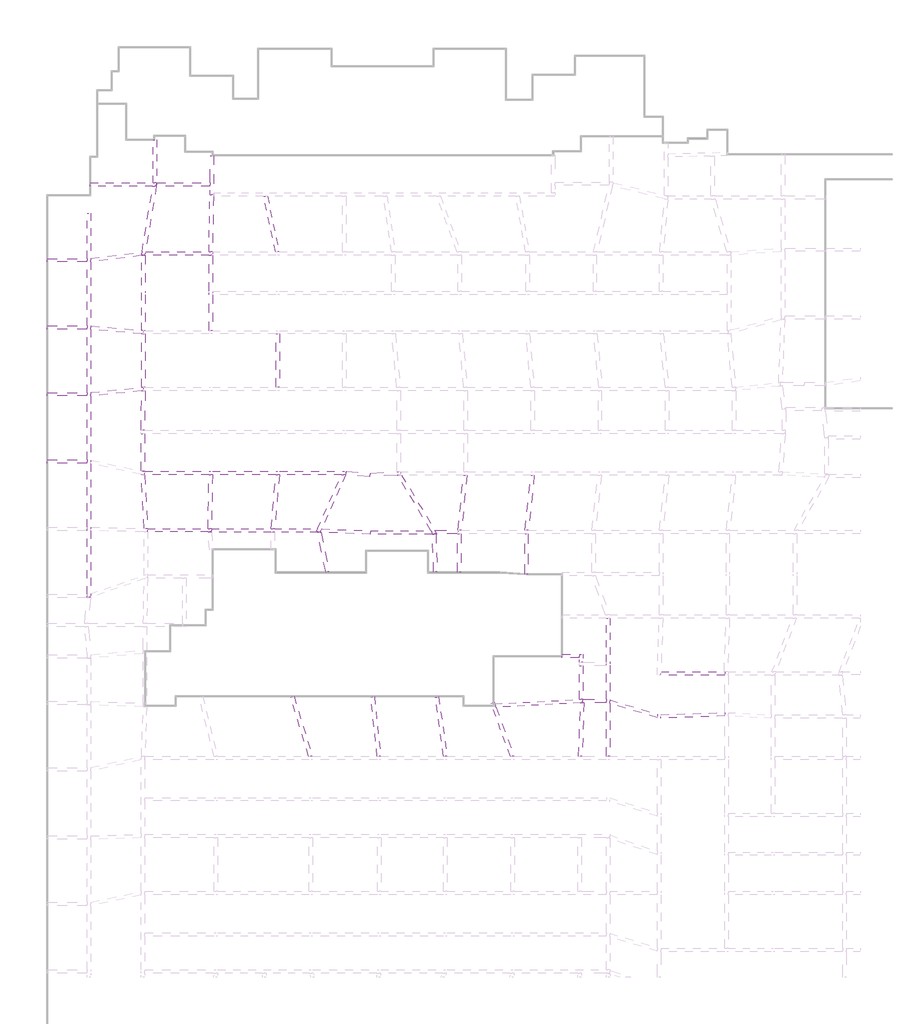
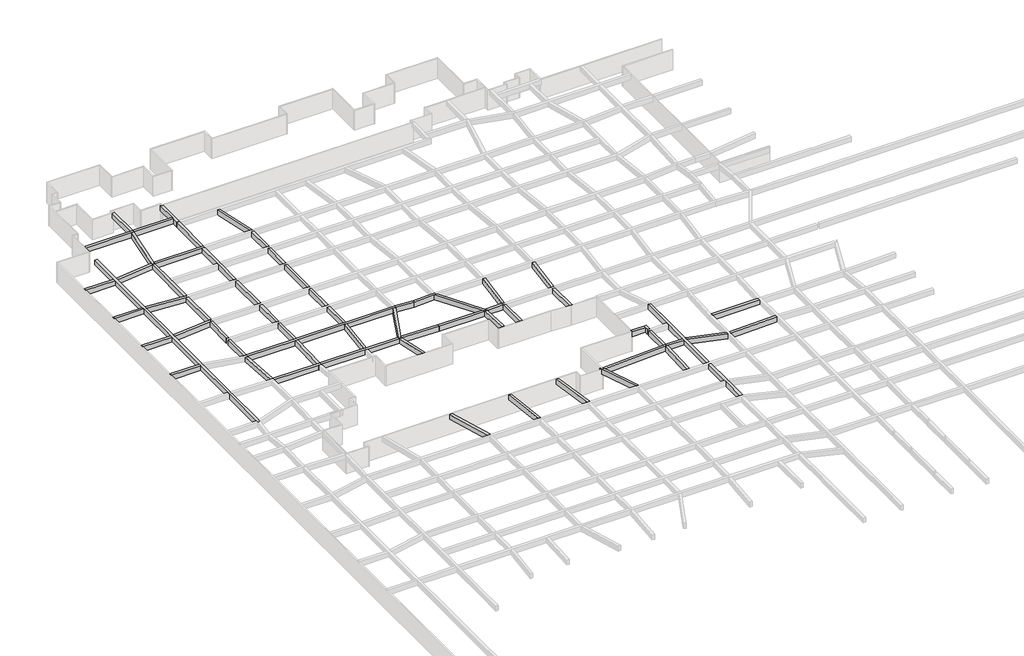
# One storey, part 35 of 45: 55 beams.
"""IFC4 building model written with IfcOpenShell, lengths in millimetres."""

from ifc_helpers import new_model, si_unit, frame, origin, place, context, project, spatial, polyline, outline, extrude, faceted_brep, element, save

model = new_model("IFC4")

# Units and contexts
model_context = context("Model", 3, world=origin())
ifc_project = project(units=[si_unit("LENGTHUNIT", "METRE", prefix="MILLI")], contexts=[model_context])

# Site, building, storey
site = spatial("IfcSite", under=ifc_project)
building = spatial("IfcBuilding", under=site)
storey = spatial("IfcBuildingStorey", under=building, Name="户型图", Elevation=0.0)

# Beams
placement = place(None, origin())
element("IfcBeam", 1, ObjectType="混凝土 - 矩形梁 : KL_beam", at=placement, inside=storey, context=model_context, shape_type="Brep", body=[
    faceted_brep([(-150040.5216564, 192731.9876735, 3300.0), (-150040.5216564, 192731.9876735, 2500.0), (-150040.5216564, 192331.9876735, 2500.0), (-150040.5216564, 192331.9876735, 3300.0), (-142370.8493457, 192331.9876735, 3300.0), (-142370.8493457, 192731.9876735, 3300.0), (-142740.5216564, 192731.9876735, 3300.0), (-142776.2701991, 192331.9876735, 3300.0), (-142370.8493457, 192331.9876735, 2500.0), (-142776.2701991, 192331.9876735, 2500.0), (-142370.8493457, 192731.9876735, 2500.0), (-142740.5216564, 192731.9876735, 2500.0)], [[[0, 1, 2, 3]], [[4, 5, 6, 0, 3, 7]], [[8, 4, 7, 3, 2, 9]], [[10, 8, 9, 2, 1, 11]], [[5, 10, 11, 1, 0, 6]], [[5, 4, 8, 10]]]),
])
element("IfcBeam", 2, ObjectType="混凝土 - 矩形梁 : KL_beam", at=placement, inside=storey, context=model_context, shape_type="Brep", body=[
    faceted_brep([(-143691.0021546, 184340.2921988, 3300.0), (-143624.9259227, 184740.2921988, 3300.0), (-142370.8493457, 192331.9876735, 3300.0), (-142776.2701991, 192331.9876735, 3300.0), (-144033.6062149, 184720.560815, 3300.0), (-144085.653783, 184405.4849301, 3300.0), (-143758.1300846, 184351.3811005, 3300.0), (-144085.653783, 184405.4849301, 2500.0), (-142776.2701991, 192331.9876735, 2500.0), (-144033.6062149, 184720.560815, 2500.0), (-142370.8493457, 192331.9876735, 2500.0), (-143624.9259227, 184740.2921988, 2500.0), (-143691.0021546, 184340.2921988, 2500.0), (-143758.1300846, 184351.3811005, 2500.0)], [[[0, 1, 2, 3, 4, 5, 6]], [[7, 5, 4, 3, 8, 9]], [[10, 11, 12, 13, 7, 9, 8]], [[2, 1, 0, 12, 11, 10]], [[3, 2, 10, 8]], [[0, 6, 5, 7, 13, 12]]]),
])
element("IfcBeam", 3, ObjectType="混凝土 - 矩形梁 : KL_beam", at=placement, inside=storey, context=model_context, shape_type="Brep", body=[
    faceted_brep([(-135864.1350128, 184340.2921988, 3300.0), (-135857.1529868, 184740.2921988, 3300.0), (-136257.213918, 184740.2921988, 3300.0), (-143624.9259227, 184740.2921988, 3300.0), (-143691.0021546, 184340.2921988, 3300.0), (-143669.0135418, 184340.2921988, 3300.0), (-136260.6744654, 184340.2921988, 3300.0), (-135864.1350128, 184340.2921988, 2500.0), (-143691.0021546, 184340.2921988, 2500.0), (-143669.0135418, 184340.2921988, 2500.0), (-136260.6744654, 184340.2921988, 2500.0), (-135857.1529868, 184740.2921988, 2500.0), (-143624.9259227, 184740.2921988, 2500.0), (-136257.213918, 184740.2921988, 2500.0)], [[[0, 1, 2, 3, 4, 5, 6]], [[7, 0, 6, 5, 4, 8, 9, 10]], [[11, 7, 10, 9, 8, 12, 13]], [[1, 11, 13, 12, 3, 2]], [[4, 3, 12, 8]], [[1, 0, 7, 11]]]),
])
element("IfcBeam", 4, ObjectType="混凝土 - 矩形梁 : KL_beam", at=placement, inside=storey, context=model_context, shape_type="Brep", body=[
    faceted_brep([(-135741.3000054, 191377.5050601, 3300.0), (-136141.3000054, 191380.9958072, 3300.0), (-136257.213918, 184740.2921988, 3300.0), (-135857.1529868, 184740.2921988, 3300.0), (-135744.7605527, 191179.2504337, 3300.0), (-135741.3000054, 191377.5050601, 2500.0), (-135857.1529868, 184740.2921988, 2500.0), (-135744.7605527, 191179.2504337, 2500.0), (-136141.3000054, 191380.9958072, 2500.0), (-136257.213918, 184740.2921988, 2500.0)], [[[0, 1, 2, 3, 4]], [[5, 0, 4, 3, 6, 7]], [[8, 5, 7, 6, 9]], [[1, 8, 9, 2]], [[3, 2, 9, 6]], [[1, 0, 5, 8]]]),
])
element("IfcBeam", 5, ObjectType="混凝土 - 矩形梁 : KL_beam", at=placement, inside=storey, context=model_context, shape_type="SweptSolid", body=[
    extrude(outline(polyline([(-128118.5648498, 184740.2921988), (-128527.5010878, 184740.2921988), (-129896.1439109, 191179.2504337), (-129487.2076729, 191179.2504337), (-128118.5648498, 184740.2921988)])), frame((0.0, 0.0, 2500.0), z_axis=(0.0, 0.0, 1.0), x_axis=(1.0, 0.0, 0.0)), (0.0, 0.0, 1.0), 800.0),
])
element("IfcBeam", 6, ObjectType="混凝土 - 矩形梁 : KL_beam", at=placement, inside=storey, context=model_context, shape_type="Brep", body=[
    faceted_brep([(-144085.653783, 184405.4849301, 3300.0), (-144033.6062149, 184720.560815, 3300.0), (-149980.0650049, 183990.4274835, 3300.0), (-149980.0650049, 183587.4235533, 3300.0), (-144069.0135418, 184313.2094117, 3300.0), (-143758.1300846, 184351.3811005, 3300.0), (-144033.6062149, 184720.560815, 2500.0), (-149980.0650049, 183990.4274835, 2500.0), (-144085.653783, 184405.4849301, 2500.0), (-143758.1300846, 184351.3811005, 2500.0), (-144069.0135418, 184313.2094117, 2500.0), (-149980.0650049, 183587.4235533, 2500.0)], [[[0, 1, 2, 3, 4, 5]], [[1, 6, 7, 2]], [[6, 8, 9, 10, 11, 7]], [[9, 5, 4, 3, 11, 10]], [[0, 8, 6, 1]], [[8, 0, 5, 9]], [[3, 2, 7, 11]]]),
])
element("IfcBeam", 7, ObjectType="混凝土 - 矩形梁 : KL_beam", at=placement, inside=storey, context=model_context, shape_type="Brep", body=[
    faceted_brep([(-149980.0650049, 189229.932653, 3300.0), (-149980.0650049, 189229.932653, 2500.0), (-150380.0650049, 189229.932653, 2500.0), (-150380.0650049, 189229.932653, 3300.0), (-150380.0650049, 144687.2740394, 3300.0), (-149980.0650049, 144687.2740394, 3300.0), (-149980.0650049, 145110.3223119, 3300.0), (-149980.0650049, 152424.9959274, 3300.0), (-149980.0650049, 152825.1148483, 3300.0), (-149980.0650049, 160182.9046895, 3300.0), (-149980.0650049, 160591.8409275, 3300.0), (-149980.0650049, 168048.193678, 3300.0), (-149980.0650049, 168450.028535, 3300.0), (-149980.0650049, 175746.0869301, 3300.0), (-149980.0650049, 176147.6148651, 3300.0), (-149980.0650049, 183587.4235533, 3300.0), (-149980.0650049, 183990.4274835, 3300.0), (-150380.0650049, 183964.3686062, 3300.0), (-150380.0650049, 183564.3686062, 3300.0), (-150380.0650049, 176164.3686062, 3300.0), (-150380.0650049, 175764.3686062, 3300.0), (-150380.0650049, 168429.932653, 3300.0), (-150380.0650049, 168029.932653, 3300.0), (-150380.0650049, 160629.932653, 3300.0), (-150380.0650049, 160229.932653, 3300.0), (-150380.0650049, 152829.932653, 3300.0), (-150380.0650049, 152429.932653, 3300.0), (-150380.0650049, 145029.932653, 3300.0), (-150380.0650049, 144687.2740394, 2500.0), (-150380.0650049, 183964.3686062, 2500.0), (-150380.0650049, 183564.3686062, 2500.0), (-150380.0650049, 176164.3686062, 2500.0), (-150380.0650049, 175764.3686062, 2500.0), (-150380.0650049, 168429.932653, 2500.0), (-150380.0650049, 168029.932653, 2500.0), (-150380.0650049, 160629.932653, 2500.0), (-150380.0650049, 160229.932653, 2500.0), (-150380.0650049, 152829.932653, 2500.0), (-150380.0650049, 152429.932653, 2500.0), (-150380.0650049, 145029.932653, 2500.0), (-149980.0650049, 144687.2740394, 2500.0), (-149980.0650049, 183990.4274835, 2500.0), (-149980.0650049, 183587.4235533, 2500.0), (-149980.0650049, 176147.6148651, 2500.0), (-149980.0650049, 175746.0869301, 2500.0), (-149980.0650049, 168450.028535, 2500.0), (-149980.0650049, 168048.193678, 2500.0), (-149980.0650049, 160591.8409275, 2500.0), (-149980.0650049, 160182.9046895, 2500.0), (-149980.0650049, 152825.1148483, 2500.0), (-149980.0650049, 152424.9959274, 2500.0), (-149980.0650049, 145110.3223119, 2500.0)], [[[0, 1, 2, 3]], [[4, 5, 6, 7, 8, 9, 10, 11, 12, 13, 14, 15, 16, 0, 3, 17, 18, 19, 20, 21, 22, 23, 24, 25, 26, 27]], [[28, 4, 27, 26, 25, 24, 23, 22, 21, 20, 19, 18, 17, 3, 2, 29, 30, 31, 32, 33, 34, 35, 36, 37, 38, 39]], [[40, 28, 39, 38, 37, 36, 35, 34, 33, 32, 31, 30, 29, 2, 1, 41, 42, 43, 44, 45, 46, 47, 48, 49, 50, 51]], [[5, 40, 51, 50, 49, 48, 47, 46, 45, 44, 43, 42, 41, 1, 0, 16, 15, 14, 13, 12, 11, 10, 9, 8, 7, 6]], [[5, 4, 28, 40]]]),
])
element("IfcBeam", 8, ObjectType="混凝土 - 矩形梁 : KL_beam", at=placement, inside=storey, context=model_context, shape_type="SweptSolid", body=[
    extrude(outline(polyline([(-155040.2933307, 183564.3686062), (-155040.2933307, 183964.3686062), (-150380.0650049, 183964.3686062), (-150380.0650049, 183564.3686062), (-155040.2933307, 183564.3686062)])), frame((0.0, 0.0, 2500.0), z_axis=(0.0, 0.0, 1.0), x_axis=(1.0, 0.0, 0.0)), (0.0, 0.0, 1.0), 800.0),
])
element("IfcBeam", 9, ObjectType="混凝土 - 矩形梁 : KL_beam", at=placement, inside=storey, context=model_context, shape_type="SweptSolid", body=[
    extrude(outline(polyline([(-155040.2933307, 175764.3686062), (-155040.2933307, 176164.3686062), (-150380.0650049, 176164.3686062), (-150380.0650049, 175764.3686062), (-155040.2933307, 175764.3686062)])), frame((0.0, 0.0, 2500.0), z_axis=(0.0, 0.0, 1.0), x_axis=(1.0, 0.0, 0.0)), (0.0, 0.0, 1.0), 800.0),
])
element("IfcBeam", 10, ObjectType="混凝土 - 矩形梁 : KL_beam", at=placement, inside=storey, context=model_context, shape_type="SweptSolid", body=[
    extrude(outline(polyline([(-155040.2933307, 168029.932653), (-155040.2933307, 168429.932653), (-150380.0650049, 168429.932653), (-150380.0650049, 168029.932653), (-155040.2933307, 168029.932653)])), frame((0.0, 0.0, 2500.0), z_axis=(0.0, 0.0, 1.0), x_axis=(1.0, 0.0, 0.0)), (0.0, 0.0, 1.0), 800.0),
])
element("IfcBeam", 11, ObjectType="混凝土 - 矩形梁 : KL_beam", at=placement, inside=storey, context=model_context, shape_type="SweptSolid", body=[
    extrude(outline(polyline([(-155040.2933307, 160229.932653), (-155040.2933307, 160629.932653), (-150380.0650049, 160629.932653), (-150380.0650049, 160229.932653), (-155040.2933307, 160229.932653)])), frame((0.0, 0.0, 2500.0), z_axis=(0.0, 0.0, 1.0), x_axis=(1.0, 0.0, 0.0)), (0.0, 0.0, 1.0), 800.0),
])
element("IfcBeam", 12, ObjectType="混凝土 - 矩形梁 : KL_beam", at=placement, inside=storey, context=model_context, shape_type="Brep", body=[
    faceted_brep([(-143913.3828558, 175215.3210168, 3300.0), (-143895.9184786, 175615.3210168, 3300.0), (-144069.0135418, 175630.4648726, 3300.0), (-149980.0650049, 176147.6148651, 3300.0), (-149980.0650049, 175746.0869301, 3300.0), (-144069.0135418, 175228.9369376, 3300.0), (-143913.3828558, 175215.3210168, 2500.0), (-149980.0650049, 175746.0869301, 2500.0), (-144069.0135418, 175228.9369376, 2500.0), (-143895.9184786, 175615.3210168, 2500.0), (-149980.0650049, 176147.6148651, 2500.0), (-144069.0135418, 175630.4648726, 2500.0)], [[[0, 1, 2, 3, 4, 5]], [[6, 0, 5, 4, 7, 8]], [[9, 6, 8, 7, 10, 11]], [[1, 9, 11, 10, 3, 2]], [[4, 3, 10, 7]], [[1, 0, 6, 9]]]),
])
element("IfcBeam", 13, ObjectType="混凝土 - 矩形梁 : KL_beam", at=placement, inside=storey, context=model_context, shape_type="Brep", body=[
    faceted_brep([(-143859.4474089, 168635.1135794, 3300.0), (-143878.581976, 169035.1135794, 3300.0), (-144069.0135418, 169016.8526647, 3300.0), (-149980.0650049, 168450.028535, 3300.0), (-149980.0650049, 168048.193678, 3300.0), (-144071.7625624, 168614.7541979, 3300.0), (-143859.4474089, 168635.1135794, 2500.0), (-149980.0650049, 168048.193678, 2500.0), (-144071.7625624, 168614.7541979, 2500.0), (-143878.581976, 169035.1135794, 2500.0), (-149980.0650049, 168450.028535, 2500.0), (-144069.0135418, 169016.8526647, 2500.0)], [[[0, 1, 2, 3, 4, 5]], [[6, 0, 5, 4, 7, 8]], [[9, 6, 8, 7, 10, 11]], [[1, 9, 11, 10, 3, 2]], [[4, 3, 10, 7]], [[1, 0, 6, 9]]]),
])
element("IfcBeam", 14, ObjectType="混凝土 - 矩形梁 : KL_beam", at=placement, inside=storey, context=model_context, shape_type="Brep", body=[
    faceted_brep([(-143391.7428195, 152664.4498776, 3300.0), (-143391.9766848, 152669.0307398, 3300.0), (-143707.512981, 158849.6325984, 3300.0), (-144112.4278844, 158935.6999181, 3300.0), (-143792.7630206, 152674.2292868, 3300.0), (-144112.4278844, 158935.6999181, 2500.0), (-143792.7630206, 152674.2292868, 2500.0), (-143707.512981, 158849.6325984, 2500.0), (-143391.9766848, 152669.0307398, 2500.0), (-143391.7428195, 152664.4498776, 2500.0)], [[[0, 1, 2, 3, 4]], [[3, 5, 6, 4]], [[7, 8, 9, 6, 5]], [[2, 1, 0, 9, 8, 7]], [[3, 2, 7, 5]], [[0, 4, 6, 9]]]),
])
element("IfcBeam", 15, ObjectType="混凝土 - 矩形梁 : KL_beam", at=placement, inside=storey, context=model_context, shape_type="Brep", body=[
    faceted_brep([(-143391.9766848, 152669.0307398, 3300.0), (-143391.7428195, 152664.4498776, 3300.0), (-143382.0266166, 152664.2129351, 3300.0), (-143382.0266166, 152269.0307398, 3300.0), (-136378.8977394, 152269.0307398, 3300.0), (-135978.8368082, 152269.0307398, 3300.0), (-135972.5274142, 152630.4956807, 3300.0), (-135971.8547822, 152669.0307398, 3300.0), (-136371.9157134, 152669.0307398, 3300.0), (-135978.8368082, 152269.0307398, 2500.0), (-143382.0266166, 152269.0307398, 2500.0), (-136378.8977394, 152269.0307398, 2500.0), (-143391.7428195, 152664.4498776, 2500.0), (-143391.9766848, 152669.0307398, 2500.0), (-136371.9157134, 152669.0307398, 2500.0), (-135971.8547822, 152669.0307398, 2500.0), (-135972.5274142, 152630.4956807, 2500.0), (-143382.0266166, 152664.2129351, 2500.0)], [[[0, 1, 2, 3, 4, 5, 6, 7, 8]], [[9, 5, 4, 3, 10, 11]], [[12, 13, 14, 15, 16, 9, 11, 10, 17]], [[13, 0, 8, 7, 15, 14]], [[1, 0, 13, 12]], [[2, 17, 10, 3]], [[17, 2, 1, 12]], [[7, 6, 5, 9, 16, 15]]]),
])
element("IfcBeam", 16, ObjectType="混凝土 - 矩形梁 : KL_beam", at=placement, inside=storey, context=model_context, shape_type="Brep", body=[
    faceted_brep([(-135860.6744654, 184340.2921988, 3300.0), (-135864.1350128, 184340.2921988, 3300.0), (-136260.6744654, 184340.2921988, 3300.0), (-136260.6744654, 180177.2946529, 3300.0), (-136260.6744654, 179777.2946529, 3300.0), (-136260.6744654, 175615.3210168, 3300.0), (-135860.6744654, 175615.3210168, 3300.0), (-135860.6744654, 179777.2946529, 3300.0), (-135860.6744654, 180177.2946529, 3300.0), (-136260.6744654, 184340.2921988, 2500.0), (-136260.6744654, 180177.2946529, 2500.0), (-136260.6744654, 179777.2946529, 2500.0), (-136260.6744654, 175615.3210168, 2500.0), (-135864.1350128, 184340.2921988, 2500.0), (-135860.6744654, 184340.2921988, 2500.0), (-135860.6744654, 180177.2946529, 2500.0), (-135860.6744654, 179777.2946529, 2500.0), (-135860.6744654, 175615.3210168, 2500.0)], [[[0, 1, 2, 3, 4, 5, 6, 7, 8]], [[2, 9, 10, 11, 12, 5, 4, 3]], [[9, 13, 14, 15, 16, 17, 12, 11, 10]], [[14, 0, 8, 7, 6, 17, 16, 15]], [[9, 2, 1, 0, 14, 13]], [[6, 5, 12, 17]]]),
    faceted_brep([(-136260.6744654, 175215.3210168, 3300.0), (-135860.6744654, 175215.3210168, 3300.0), (-135860.6744654, 175215.3210168, 2500.0), (-136260.6744654, 175215.3210168, 2500.0), (-135860.6744654, 169035.1135794, 3300.0), (-136260.6744654, 169035.1135794, 3300.0), (-136260.6744654, 169035.1135794, 2500.0), (-135860.6744654, 169035.1135794, 2500.0)], [[[0, 1, 2, 3]], [[4, 5, 6, 7]], [[1, 0, 5, 4]], [[0, 3, 6, 5]], [[3, 2, 7, 6]], [[2, 1, 4, 7]]]),
    faceted_brep([(-135860.6744654, 168635.1135794, 3300.0), (-136260.6744654, 168635.1135794, 3300.0), (-136260.6744654, 164050.6823883, 3300.0), (-135860.6744654, 164050.6823883, 3300.0), (-136260.6744654, 168635.1135794, 2500.0), (-136260.6744654, 164050.6823883, 2500.0), (-135860.6744654, 168635.1135794, 2500.0), (-135860.6744654, 164050.6823883, 2500.0)], [[[0, 1, 2, 3]], [[1, 4, 5, 2]], [[4, 6, 7, 5]], [[6, 0, 3, 7]], [[1, 0, 6, 4]], [[3, 2, 5, 7]]]),
    faceted_brep([(-136260.6744654, 163650.6823883, 3300.0), (-135860.6744654, 163650.6823883, 3300.0), (-135860.6744654, 163650.6823883, 2500.0), (-136260.6744654, 163650.6823883, 2500.0), (-136260.6744654, 159299.3775215, 3300.0), (-135860.6744654, 159299.3775215, 3300.0), (-136260.6744654, 159299.3775215, 2500.0), (-135860.6744654, 159299.3775215, 2500.0)], [[[0, 1, 2, 3]], [[1, 0, 4, 5]], [[0, 3, 6, 4]], [[3, 2, 7, 6]], [[2, 1, 5, 7]], [[5, 4, 6, 7]]]),
])
element("IfcBeam", 17, ObjectType="混凝土 - 矩形梁 : KL_beam", at=placement, inside=storey, context=model_context, shape_type="SweptSolid", body=[
    extrude(outline(polyline([(-135971.8547822, 152669.0307398), (-136371.9157134, 152669.0307398), (-136263.1646058, 158899.3775215), (-135863.1036746, 158899.3775215), (-135971.8547822, 152669.0307398)])), frame((0.0, 0.0, 2500.0), z_axis=(0.0, 0.0, 1.0), x_axis=(1.0, 0.0, 0.0)), (0.0, 0.0, 1.0), 800.0),
])
element("IfcBeam", 18, ObjectType="混凝土 - 矩形梁 : KL_beam", at=placement, inside=storey, context=model_context, shape_type="Brep", body=[
    faceted_brep([(-143899.5027499, 159299.3775215, 3300.0), (-143728.6193094, 159263.055125, 3300.0), (-143710.0525927, 158899.3775215, 3300.0), (-136263.1646058, 158899.3775215, 3300.0), (-135863.1036746, 158899.3775215, 3300.0), (-128498.7833567, 158899.3775215, 3300.0), (-128097.2554216, 158899.3775215, 3300.0), (-120868.6474581, 158899.3775215, 3300.0), (-120430.7929467, 158899.3775215, 3300.0), (-120360.6744654, 159056.8662092, 3300.0), (-120360.6744654, 159285.8508502, 3300.0), (-120360.6744654, 159299.3775215, 3300.0), (-120760.6744654, 159299.3775215, 3300.0), (-128080.5216564, 159299.3775215, 3300.0), (-128480.5216564, 159299.3775215, 3300.0), (-135860.6744654, 159299.3775215, 3300.0), (-136260.6744654, 159299.3775215, 3300.0), (-143730.8224936, 159299.3775215, 3300.0), (-143710.0525927, 158899.3775215, 2500.0), (-136263.1646058, 158899.3775215, 2500.0), (-135863.1036746, 158899.3775215, 2500.0), (-128498.7833567, 158899.3775215, 2500.0), (-128097.2554216, 158899.3775215, 2500.0), (-120868.6474581, 158899.3775215, 2500.0), (-120430.7929467, 158899.3775215, 2500.0), (-143728.6193094, 159263.055125, 2500.0), (-143899.5027499, 159299.3775215, 2500.0), (-143730.8224936, 159299.3775215, 2500.0), (-136260.6744654, 159299.3775215, 2500.0), (-135860.6744654, 159299.3775215, 2500.0), (-128480.5216564, 159299.3775215, 2500.0), (-128080.5216564, 159299.3775215, 2500.0), (-120760.6744654, 159299.3775215, 2500.0), (-120360.6744654, 159299.3775215, 2500.0), (-120360.6744654, 159285.8508502, 2500.0), (-120360.6744654, 159056.8662092, 2500.0)], [[[0, 1, 2, 3, 4, 5, 6, 7, 8, 9, 10, 11, 12, 13, 14, 15, 16, 17]], [[2, 18, 19, 20, 21, 22, 23, 24, 8, 7, 6, 5, 4, 3]], [[25, 26, 27, 28, 29, 30, 31, 32, 33, 34, 35, 24, 23, 22, 21, 20, 19, 18]], [[26, 0, 17, 16, 15, 14, 13, 12, 11, 33, 32, 31, 30, 29, 28, 27]], [[25, 1, 0, 26]], [[1, 25, 18, 2]], [[11, 10, 9, 35, 34, 33]], [[35, 9, 8, 24]]]),
])
element("IfcBeam", 19, ObjectType="混凝土 - 矩形梁 : KL_beam", at=placement, inside=storey, context=model_context, shape_type="SweptSolid", body=[
    extrude(outline(polyline([(-144130.8224936, 163650.6823883), (-143730.8224936, 163650.6823883), (-143730.8224936, 159299.3775215), (-143899.5027499, 159299.3775215), (-144130.8224936, 159348.5460509), (-144130.8224936, 163650.6823883)])), frame((0.0, 0.0, 2500.0), z_axis=(0.0, 0.0, 1.0), x_axis=(1.0, 0.0, 0.0)), (0.0, 0.0, 1.0), 800.0),
])
element("IfcBeam", 20, ObjectType="混凝土 - 矩形梁 : KL_beam", at=placement, inside=storey, context=model_context, shape_type="SweptSolid", body=[
    extrude(outline(polyline([(-144071.7625624, 168614.7541979), (-143859.4474089, 168635.1135794), (-143671.4793509, 168635.1135794), (-143728.3270835, 164050.6823883), (-144128.3578352, 164050.6823883), (-144071.7625624, 168614.7541979)])), frame((0.0, 0.0, 2500.0), z_axis=(0.0, 0.0, 1.0), x_axis=(1.0, 0.0, 0.0)), (0.0, 0.0, 1.0), 800.0),
])
element("IfcBeam", 21, ObjectType="混凝土 - 矩形梁 : KL_beam", at=placement, inside=storey, context=model_context, shape_type="Brep", body=[
    faceted_brep([(-143878.581976, 169035.1135794, 3300.0), (-143669.0135418, 169035.1135794, 3300.0), (-143669.0135418, 175215.3210168, 3300.0), (-143913.3828558, 175215.3210168, 3300.0), (-144069.0135418, 175228.9369376, 3300.0), (-144069.0135418, 169016.8526647, 3300.0), (-144066.7738093, 169017.0674377, 3300.0), (-143669.0135418, 169035.1135794, 2500.0), (-143669.0135418, 175215.3210168, 2500.0), (-143878.581976, 169035.1135794, 2500.0), (-144066.7738093, 169017.0674377, 2500.0), (-144069.0135418, 169016.8526647, 2500.0), (-144069.0135418, 175228.9369376, 2500.0), (-143913.3828558, 175215.3210168, 2500.0)], [[[0, 1, 2, 3, 4, 5, 6]], [[1, 7, 8, 2]], [[7, 9, 10, 11, 12, 13, 8]], [[4, 12, 11, 5]], [[1, 0, 9, 7]], [[3, 2, 8, 13]], [[4, 3, 13, 12]], [[5, 11, 10, 9, 0, 6]]]),
])
element("IfcBeam", 22, ObjectType="混凝土 - 矩形梁 : KL_beam", at=placement, inside=storey, context=model_context, shape_type="Brep", body=[
    faceted_brep([(-143895.9184786, 175615.3210168, 3300.0), (-143669.0135418, 175615.3210168, 3300.0), (-143669.0135418, 179777.2946529, 3300.0), (-143669.0135418, 180177.2946529, 3300.0), (-143669.0135418, 184340.2921988, 3300.0), (-143691.0021546, 184340.2921988, 3300.0), (-143758.1300846, 184351.3811005, 3300.0), (-144069.0135418, 184313.2094117, 3300.0), (-144069.0135418, 175630.4648726, 3300.0), (-143669.0135418, 175615.3210168, 2500.0), (-143669.0135418, 179777.2946529, 2500.0), (-143669.0135418, 180177.2946529, 2500.0), (-143669.0135418, 184340.2921988, 2500.0), (-143895.9184786, 175615.3210168, 2500.0), (-144069.0135418, 175630.4648726, 2500.0), (-144069.0135418, 184313.2094117, 2500.0), (-143758.1300846, 184351.3811005, 2500.0), (-143691.0021546, 184340.2921988, 2500.0)], [[[0, 1, 2, 3, 4, 5, 6, 7, 8]], [[1, 9, 10, 11, 12, 4, 3, 2]], [[9, 13, 14, 15, 16, 17, 12, 11, 10]], [[7, 15, 14, 8]], [[1, 0, 13, 9]], [[15, 7, 6, 16]], [[6, 5, 17, 16]], [[5, 4, 12, 17]], [[0, 8, 14, 13]]]),
])
element("IfcBeam", 23, ObjectType="混凝土 - 矩形梁 : KL_beam", at=placement, inside=storey, context=model_context, shape_type="SweptSolid", body=[
    extrude(outline(polyline([(-128480.5216564, 184340.2921988), (-128080.5216564, 184340.2921988), (-128080.5216564, 180177.2946529), (-128480.5216564, 180177.2946529), (-128480.5216564, 184340.2921988)])), frame((0.0, 0.0, 2500.0), z_axis=(0.0, 0.0, 1.0), x_axis=(1.0, 0.0, 0.0)), (0.0, 0.0, 1.0), 800.0),
    extrude(outline(polyline([(-128080.5216564, 159299.3775215), (-128480.5216564, 159299.3775215), (-128480.5216564, 163650.6823883), (-128080.5216564, 163650.6823883), (-128080.5216564, 159299.3775215)])), frame((0.0, 0.0, 2500.0), z_axis=(0.0, 0.0, 1.0), x_axis=(1.0, 0.0, 0.0)), (0.0, 0.0, 1.0), 800.0),
    extrude(outline(polyline([(-128480.5216564, 175215.3210168), (-128080.5216564, 175215.3210168), (-128080.5216564, 169035.1135794), (-128480.5216564, 169035.1135794), (-128480.5216564, 175215.3210168)])), frame((0.0, 0.0, 2500.0), z_axis=(0.0, 0.0, 1.0), x_axis=(1.0, 0.0, 0.0)), (0.0, 0.0, 1.0), 800.0),
    extrude(outline(polyline([(-128080.5216564, 175615.3210168), (-128480.5216564, 175615.3210168), (-128480.5216564, 179777.2946529), (-128080.5216564, 179777.2946529), (-128080.5216564, 175615.3210168)])), frame((0.0, 0.0, 2500.0), z_axis=(0.0, 0.0, 1.0), x_axis=(1.0, 0.0, 0.0)), (0.0, 0.0, 1.0), 800.0),
    extrude(outline(polyline([(-128480.5216564, 168635.1135794), (-128080.5216564, 168635.1135794), (-128080.5216564, 164050.6823883), (-128480.5216564, 164050.6823883), (-128480.5216564, 168635.1135794)])), frame((0.0, 0.0, 2500.0), z_axis=(0.0, 0.0, 1.0), x_axis=(1.0, 0.0, 0.0)), (0.0, 0.0, 1.0), 800.0),
])
element("IfcBeam", 24, ObjectType="混凝土 - 矩形梁 : KL_beam", at=placement, inside=storey, context=model_context, shape_type="SweptSolid", body=[
    extrude(outline(polyline([(-128498.7833567, 158899.3775215), (-128097.2554216, 158899.3775215), (-128645.7115157, 152630.4956807), (-129047.2394507, 152630.4956807), (-128498.7833567, 158899.3775215)])), frame((0.0, 0.0, 2500.0), z_axis=(0.0, 0.0, 1.0), x_axis=(1.0, 0.0, 0.0)), (0.0, 0.0, 1.0), 800.0),
])
element("IfcBeam", 25, ObjectType="混凝土 - 矩形梁 : KL_beam", at=placement, inside=storey, context=model_context, shape_type="Brep", body=[
    faceted_brep([(-123767.4305173, 152388.604171, 3300.0), (-123412.3130339, 152230.4956807, 3300.0), (-123402.0123343, 152225.9095138, 3300.0), (-123226.540494, 152620.0257198, 3300.0), (-120434.9382056, 158890.0671176, 3300.0), (-120430.7929467, 158899.3775215, 3300.0), (-120868.6474581, 158899.3775215, 3300.0), (-123659.7334785, 152630.4956807, 3300.0), (-123767.4305173, 152388.604171, 2500.0), (-120868.6474581, 158899.3775215, 2500.0), (-123659.7334785, 152630.4956807, 2500.0), (-123402.0123343, 152225.9095138, 2500.0), (-123412.3130339, 152230.4956807, 2500.0), (-120430.7929467, 158899.3775215, 2500.0), (-120434.9382056, 158890.0671176, 2500.0), (-123226.540494, 152620.0257198, 2500.0)], [[[0, 1, 2, 3, 4, 5, 6, 7]], [[8, 0, 7, 6, 9, 10]], [[11, 12, 8, 10, 9, 13, 14, 15]], [[2, 11, 15, 14, 13, 5, 4, 3]], [[6, 5, 13, 9]], [[2, 1, 0, 8, 12, 11]]]),
])
element("IfcBeam", 26, ObjectType="混凝土 - 矩形梁 : KL_beam", at=placement, inside=storey, context=model_context, shape_type="Brep", body=[
    faceted_brep([(-117566.6583118, 159090.4742081, 3300.0), (-120360.6744654, 159285.8508502, 3300.0), (-120360.6744654, 159056.8662092, 3300.0), (-120430.7929467, 158899.3775215, 3300.0), (-120434.9382056, 158890.0671176, 3300.0), (-117570.1554489, 158689.7419925, 3300.0), (-120434.9382056, 158890.0671176, 2500.0), (-117570.1554489, 158689.7419925, 2500.0), (-120430.7929467, 158899.3775215, 2500.0), (-120360.6744654, 159056.8662092, 2500.0), (-120360.6744654, 159285.8508502, 2500.0), (-117566.6583118, 159090.4742081, 2500.0)], [[[0, 1, 2, 3, 4, 5]], [[5, 4, 6, 7]], [[7, 6, 8, 9, 10, 11]], [[1, 0, 11, 10]], [[2, 9, 8, 6, 4, 3]], [[9, 2, 1, 10]], [[0, 5, 7, 11]]]),
])
element("IfcBeam", 27, ObjectType="混凝土 - 矩形梁 : KL_beam", at=placement, inside=storey, context=model_context, shape_type="Brep", body=[
    faceted_brep([(-117566.6583118, 159090.4742081, 3300.0), (-117570.1554489, 158689.7419925, 3300.0), (-114382.4696565, 158856.8015259, 3300.0), (-114259.4336062, 158863.2495721, 3300.0), (-114072.9294157, 158873.0238425, 3300.0), (-114072.9294157, 159263.2495721, 3300.0), (-114072.9294157, 159273.5727809, 3300.0), (-114472.9294157, 159252.6096692, 3300.0), (-117570.1554489, 158689.7419925, 2500.0), (-114382.4696565, 158856.8015259, 2500.0), (-114259.4336062, 158863.2495721, 2500.0), (-114072.9294157, 158873.0238425, 2500.0), (-117566.6583118, 159090.4742081, 2500.0), (-114472.9294157, 159252.6096692, 2500.0), (-114072.9294157, 159273.5727809, 2500.0), (-114072.9294157, 159263.2495721, 2500.0)], [[[0, 1, 2, 3, 4, 5, 6, 7]], [[1, 8, 9, 10, 11, 4, 3, 2]], [[8, 12, 13, 14, 15, 11, 10, 9]], [[12, 0, 7, 6, 14, 13]], [[0, 12, 8, 1]], [[6, 5, 4, 11, 15, 14]]]),
])
element("IfcBeam", 28, ObjectType="混凝土 - 矩形梁 : KL_beam", at=placement, inside=storey, context=model_context, shape_type="Brep", body=[
    faceted_brep([(-110310.4324421, 152079.7935386, 3300.0), (-109843.7790832, 152079.7935386, 3300.0), (-110084.1233308, 152479.7935386, 3300.0), (-113919.6906746, 158863.2495721, 3300.0), (-114259.4336062, 158863.2495721, 3300.0), (-114382.4696565, 158856.8015259, 3300.0), (-110515.509273, 152421.0987005, 3300.0), (-114382.4696565, 158856.8015259, 2500.0), (-110515.509273, 152421.0987005, 2500.0), (-110310.4324421, 152079.7935386, 2500.0), (-109843.7790832, 152079.7935386, 2500.0), (-114259.4336062, 158863.2495721, 2500.0), (-113919.6906746, 158863.2495721, 2500.0), (-110084.1233308, 152479.7935386, 2500.0)], [[[0, 1, 2, 3, 4, 5, 6]], [[5, 7, 8, 9, 0, 6]], [[10, 9, 8, 7, 11, 12, 13]], [[1, 10, 13, 12, 3, 2]], [[7, 5, 4, 11]], [[4, 3, 12, 11]], [[1, 0, 9, 10]]]),
])
element("IfcBeam", 29, ObjectType="混凝土 - 矩形梁 : KL_beam", at=placement, inside=storey, context=model_context, shape_type="Brep", body=[
    faceted_brep([(-110084.1233308, 152479.7935386, 3300.0), (-109843.7790832, 152079.7935386, 3300.0), (-107419.2456688, 152079.7935386, 3300.0), (-107399.1449794, 152079.7935386, 3300.0), (-107399.1449794, 152479.7935386, 3300.0), (-110084.1233308, 152479.7935386, 2500.0), (-107399.1449794, 152479.7935386, 2500.0), (-109843.7790832, 152079.7935386, 2500.0), (-107399.1449794, 152079.7935386, 2500.0), (-107419.2456688, 152079.7935386, 2500.0)], [[[0, 1, 2, 3, 4]], [[5, 0, 4, 6]], [[7, 5, 6, 8, 9]], [[1, 7, 9, 8, 3, 2]], [[1, 0, 5, 7]], [[4, 3, 8, 6]]]),
])
element("IfcBeam", 30, ObjectType="混凝土 - 矩形梁 : KL_beam", at=placement, inside=storey, context=model_context, shape_type="SweptSolid", body=[
    extrude(outline(polyline([(-106996.9062488, 152479.7935386), (-107399.1449794, 152479.7935386), (-106722.8306205, 158863.2495721), (-106320.5918899, 158863.2495721), (-106996.9062488, 152479.7935386)])), frame((0.0, 0.0, 2500.0), z_axis=(0.0, 0.0, 1.0), x_axis=(1.0, 0.0, 0.0)), (0.0, 0.0, 1.0), 800.0),
])
element("IfcBeam", 31, ObjectType="混凝土 - 矩形梁 : KL_beam", at=placement, inside=storey, context=model_context, shape_type="SweptSolid", body=[
    extrude(outline(polyline([(-98947.1541949, 158863.2495721), (-98544.9154643, 158863.2495721), (-99221.2298232, 152479.7935386), (-99623.4685538, 152479.7935386), (-98947.1541949, 158863.2495721)])), frame((0.0, 0.0, 2500.0), z_axis=(0.0, 0.0, 1.0), x_axis=(1.0, 0.0, 0.0)), (0.0, 0.0, 1.0), 800.0),
])
element("IfcBeam", 32, ObjectType="混凝土 - 矩形梁 : KL_beam", at=placement, inside=storey, context=model_context, shape_type="Brep", body=[
    faceted_brep([(-123402.0123343, 152225.9095138, 3300.0), (-123281.0986767, 152221.6871158, 3300.0), (-117536.9980107, 152021.0987005, 3300.0), (-117530.0159847, 152421.0987005, 3300.0), (-123226.540494, 152620.0257198, 3300.0), (-123402.0123343, 152225.9095138, 2500.0), (-123281.0986767, 152221.6871158, 2500.0), (-117536.9980107, 152021.0987005, 2500.0), (-123226.540494, 152620.0257198, 2500.0), (-117530.0159847, 152421.0987005, 2500.0)], [[[0, 1, 2, 3, 4]], [[2, 1, 0, 5, 6, 7]], [[7, 6, 5, 8, 9]], [[3, 9, 8, 4]], [[0, 4, 8, 5]], [[3, 2, 7, 9]]]),
])
element("IfcBeam", 33, ObjectType="混凝土 - 矩形梁 : KL_beam", at=placement, inside=storey, context=model_context, shape_type="Brep", body=[
    faceted_brep([(-117536.9980107, 152021.0987005, 3300.0), (-110355.0940815, 152021.0987005, 3300.0), (-109954.8502638, 152021.0987005, 3300.0), (-109808.5116665, 152021.0987005, 3300.0), (-109843.7790832, 152079.7935386, 3300.0), (-110310.4324421, 152079.7935386, 3300.0), (-110515.509273, 152421.0987005, 3300.0), (-117530.0159847, 152421.0987005, 3300.0), (-117536.9980107, 152021.0987005, 2500.0), (-110355.0940815, 152021.0987005, 2500.0), (-109954.8502638, 152021.0987005, 2500.0), (-109808.5116665, 152021.0987005, 2500.0), (-117530.0159847, 152421.0987005, 2500.0), (-110515.509273, 152421.0987005, 2500.0), (-110310.4324421, 152079.7935386, 2500.0), (-109843.7790832, 152079.7935386, 2500.0)], [[[0, 1, 2, 3, 4, 5, 6, 7]], [[3, 2, 1, 0, 8, 9, 10, 11]], [[11, 10, 9, 8, 12, 13, 14, 15]], [[12, 7, 6, 13]], [[3, 11, 15, 4]], [[7, 12, 8, 0]], [[5, 14, 13, 6]], [[14, 5, 4, 15]]]),
])
element("IfcBeam", 34, ObjectType="混凝土 - 矩形梁 : KL_beam", at=placement, inside=storey, context=model_context, shape_type="Brep", body=[
    faceted_brep([(-136378.8977394, 152269.0307398, 3300.0), (-136379.5703714, 152230.4956807, 3300.0), (-136359.3151276, 152230.4956807, 3300.0), (-135957.7871926, 152230.4956807, 3300.0), (-129064.001285, 152230.4956807, 3300.0), (-128664.001285, 152230.4956807, 3300.0), (-123691.9072329, 152230.4956807, 3300.0), (-123412.3130339, 152230.4956807, 3300.0), (-123767.4305173, 152388.604171, 3300.0), (-123659.7334785, 152630.4956807, 3300.0), (-128645.7115157, 152630.4956807, 3300.0), (-129047.2394507, 152630.4956807, 3300.0), (-135972.5274142, 152630.4956807, 3300.0), (-135978.8368082, 152269.0307398, 3300.0), (-135972.5274142, 152630.4956807, 2500.0), (-123659.7334785, 152630.4956807, 2500.0), (-128645.7115157, 152630.4956807, 2500.0), (-129047.2394507, 152630.4956807, 2500.0), (-136379.5703714, 152230.4956807, 2500.0), (-136378.8977394, 152269.0307398, 2500.0), (-135978.8368082, 152269.0307398, 2500.0), (-123767.4305173, 152388.604171, 2500.0), (-123412.3130339, 152230.4956807, 2500.0), (-123691.9072329, 152230.4956807, 2500.0), (-128664.001285, 152230.4956807, 2500.0), (-129064.001285, 152230.4956807, 2500.0), (-135957.7871926, 152230.4956807, 2500.0), (-136359.3151276, 152230.4956807, 2500.0)], [[[0, 1, 2, 3, 4, 5, 6, 7, 8, 9, 10, 11, 12, 13]], [[14, 12, 11, 10, 9, 15, 16, 17]], [[18, 19, 20, 14, 17, 16, 15, 21, 22, 23, 24, 25, 26, 27]], [[1, 18, 27, 26, 25, 24, 23, 22, 7, 6, 5, 4, 3, 2]], [[18, 1, 0, 19]], [[13, 20, 19, 0]], [[20, 13, 12, 14]], [[8, 21, 15, 9]], [[21, 8, 7, 22]]]),
])
element("IfcBeam", 35, ObjectType="混凝土 - 矩形梁 : KL_beam", at=placement, inside=storey, context=model_context, shape_type="SweptSolid", body=[
    extrude(outline(polyline([(-122315.5536211, 147679.1547753), (-122706.8126614, 147595.990099), (-123691.9072329, 152230.4956807), (-123412.3130339, 152230.4956807), (-123402.0123343, 152225.9095138), (-123281.0986767, 152221.6871158), (-122315.5536211, 147679.1547753)])), frame((0.0, 0.0, 2500.0), z_axis=(0.0, 0.0, 1.0), x_axis=(1.0, 0.0, 0.0)), (0.0, 0.0, 1.0), 800.0),
])
element("IfcBeam", 36, ObjectType="混凝土 - 矩形梁 : KL_beam", at=placement, inside=storey, context=model_context, shape_type="SweptSolid", body=[
    extrude(outline(polyline([(-109802.9475348, 147671.173679), (-110202.7038656, 147657.2138803), (-110355.0940815, 152021.0987005), (-109954.8502638, 152021.0987005), (-109802.9475348, 147671.173679)])), frame((0.0, 0.0, 2500.0), z_axis=(0.0, 0.0, 1.0), x_axis=(1.0, 0.0, 0.0)), (0.0, 0.0, 1.0), 800.0),
])
element("IfcBeam", 37, ObjectType="混凝土 - 矩形梁 : KL_beam", at=placement, inside=storey, context=model_context, shape_type="Brep", body=[
    faceted_brep([(-107019.2456688, 147579.6498079, 3300.0), (-107419.2456688, 147579.6498079, 3300.0), (-107419.2456688, 147579.6498079, 2500.0), (-107019.2456688, 147579.6498079, 2500.0), (-107019.2456688, 152079.7935386, 3300.0), (-107399.1449794, 152079.7935386, 3300.0), (-107419.2456688, 152079.7935386, 3300.0), (-107419.2456688, 152079.7935386, 2500.0), (-107399.1449794, 152079.7935386, 2500.0), (-107019.2456688, 152079.7935386, 2500.0)], [[[0, 1, 2, 3]], [[1, 0, 4, 5, 6]], [[2, 1, 6, 7]], [[3, 2, 7, 8, 9]], [[0, 3, 9, 4]], [[7, 6, 5, 4, 9, 8]]]),
])
element("IfcBeam", 38, ObjectType="混凝土 - 矩形梁 : KL_beam", at=placement, inside=storey, context=model_context, shape_type="SweptSolid", body=[
    extrude(outline(polyline([(-99243.5692432, 147379.6498079), (-99643.5692432, 147379.6498079), (-99643.5692432, 152079.7935386), (-99243.5692432, 152079.7935386), (-99243.5692432, 147379.6498079)])), frame((0.0, 0.0, 2500.0), z_axis=(0.0, 0.0, 1.0), x_axis=(1.0, 0.0, 0.0)), (0.0, 0.0, 1.0), 800.0),
])
element("IfcBeam", 39, ObjectType="混凝土 - 矩形梁 : KL_beam", at=placement, inside=storey, context=model_context, shape_type="Brep", body=[
    faceted_brep([(-142740.5216564, 197711.9876735, 3300.0), (-142340.5216564, 197711.9876735, 3300.0), (-142340.5216564, 197711.9876735, 2500.0), (-142740.5216564, 197711.9876735, 2500.0), (-142740.5216564, 192731.9876735, 3300.0), (-142710.1939672, 192731.9876735, 3300.0), (-142370.8493457, 192731.9876735, 3300.0), (-142370.8493457, 192331.9876735, 3300.0), (-142340.5216564, 192331.9876735, 3300.0), (-142340.5216564, 192731.9876735, 3300.0), (-142340.5216564, 192331.9876735, 2500.0), (-142340.5216564, 192731.9876735, 2500.0), (-142370.8493457, 192331.9876735, 2500.0), (-142370.8493457, 192731.9876735, 2500.0), (-142710.1939672, 192731.9876735, 2500.0), (-142740.5216564, 192731.9876735, 2500.0)], [[[0, 1, 2, 3]], [[1, 0, 4, 5, 6, 7, 8, 9]], [[2, 1, 9, 8, 10, 11]], [[3, 2, 11, 10, 12, 13, 14, 15]], [[0, 3, 15, 4]], [[13, 6, 5, 4, 15, 14]], [[6, 13, 12, 7]], [[10, 8, 7, 12]]]),
])
element("IfcBeam", 40, ObjectType="混凝土 - 矩形梁 : KL_beam", at=placement, inside=storey, context=model_context, shape_type="SweptSolid", body=[
    extrude(outline(polyline([(-142340.5216564, 192331.9876735), (-142340.5216564, 192731.9876735), (-136141.3000054, 192731.9876735), (-136141.3000054, 192331.9876735), (-142340.5216564, 192331.9876735)])), frame((0.0, 0.0, 2500.0), z_axis=(0.0, 0.0, 1.0), x_axis=(1.0, 0.0, 0.0)), (0.0, 0.0, 1.0), 800.0),
])
element("IfcBeam", 41, ObjectType="混凝土 - 矩形梁 : KL_beam", at=placement, inside=storey, context=model_context, shape_type="Brep", body=[
    faceted_brep([(-136141.3000054, 195879.2504337, 3300.0), (-135741.3000054, 195879.2504337, 3300.0), (-135741.3000054, 195879.2504337, 2500.0), (-136141.3000054, 195879.2504337, 2500.0), (-136141.3000054, 192731.9876735, 3300.0), (-136141.3000054, 192331.9876735, 3300.0), (-136141.3000054, 191380.9958072, 3300.0), (-135741.3000054, 191377.5050601, 3300.0), (-135741.3000054, 191579.2504337, 3300.0), (-135741.3000054, 191377.5050601, 2500.0), (-135741.3000054, 191579.2504337, 2500.0), (-136141.3000054, 191380.9958072, 2500.0), (-136141.3000054, 192331.9876735, 2500.0), (-136141.3000054, 192731.9876735, 2500.0)], [[[0, 1, 2, 3]], [[1, 0, 4, 5, 6, 7, 8]], [[2, 1, 8, 7, 9, 10]], [[3, 2, 10, 9, 11, 12, 13]], [[0, 3, 13, 12, 11, 6, 5, 4]], [[6, 11, 9, 7]]]),
])
element("IfcBeam", 42, ObjectType="混凝土 - 矩形梁 : KL_beam", at=placement, inside=storey, context=model_context, shape_type="Brep", body=[
    faceted_brep([(-90189.4148055, 116812.9362228, 3300.0), (-89789.4148055, 116812.9362228, 3300.0), (-89789.4148055, 121019.6279557, 3300.0), (-89789.4148055, 121437.9046583, 3300.0), (-89789.4148055, 125889.9393475, 3300.0), (-90189.4148055, 125889.9393475, 3300.0), (-90189.4148055, 121489.9393475, 3300.0), (-90189.4148055, 121089.9393475, 3300.0), (-89789.4148055, 116812.9362228, 2500.0), (-89789.4148055, 121019.6279557, 2500.0), (-89789.4148055, 121437.9046583, 2500.0), (-89789.4148055, 125889.9393475, 2500.0), (-90189.4148055, 116812.9362228, 2500.0), (-90189.4148055, 121089.9393475, 2500.0), (-90189.4148055, 121489.9393475, 2500.0), (-90189.4148055, 125889.9393475, 2500.0)], [[[0, 1, 2, 3, 4, 5, 6, 7]], [[1, 8, 9, 10, 11, 4, 3, 2]], [[8, 12, 13, 14, 15, 11, 10, 9]], [[12, 0, 7, 6, 5, 15, 14, 13]], [[1, 0, 12, 8]], [[5, 4, 11, 15]]]),
    faceted_brep([(-89789.4148055, 126289.9393475, 3300.0), (-90189.4148055, 126289.9393475, 3300.0), (-90189.4148055, 126289.9393475, 2500.0), (-89789.4148055, 126289.9393475, 2500.0), (-89789.4148055, 132414.2467314, 3300.0), (-89789.4148055, 132832.523434, 3300.0), (-89789.4148055, 136800.4456596, 3300.0), (-89789.4148055, 137208.4081813, 3300.0), (-89789.4148055, 142284.531219, 3300.0), (-90189.4148055, 142284.531219, 3300.0), (-90189.4148055, 137184.531219, 3300.0), (-90189.4148055, 136784.531219, 3300.0), (-90189.4148055, 132874.6334047, 3300.0), (-90189.4148055, 132474.6334047, 3300.0), (-89789.4148055, 132414.2467314, 2500.0), (-89789.4148055, 132832.523434, 2500.0), (-89789.4148055, 136800.4456596, 2500.0), (-89789.4148055, 137208.4081813, 2500.0), (-89789.4148055, 142284.531219, 2500.0), (-90189.4148055, 132474.6334047, 2500.0), (-90189.4148055, 132874.6334047, 2500.0), (-90189.4148055, 136784.531219, 2500.0), (-90189.4148055, 137184.531219, 2500.0), (-90189.4148055, 142284.531219, 2500.0)], [[[0, 1, 2, 3]], [[1, 0, 4, 5, 6, 7, 8, 9, 10, 11, 12, 13]], [[0, 3, 14, 15, 16, 17, 18, 8, 7, 6, 5, 4]], [[3, 2, 19, 20, 21, 22, 23, 18, 17, 16, 15, 14]], [[2, 1, 13, 12, 11, 10, 9, 23, 22, 21, 20, 19]], [[9, 8, 18, 23]]]),
])
element("IfcBeam", 43, ObjectType="混凝土 - 矩形梁 : KL_beam", at=placement, inside=storey, context=model_context, shape_type="SweptSolid", body=[
    extrude(outline(polyline([(-89789.4148055, 132414.2467314), (-89789.4148055, 132832.523434), (-84261.6804358, 131142.5254383), (-84261.6804358, 130724.2487357), (-89789.4148055, 132414.2467314)])), frame((0.0, 0.0, 2500.0), z_axis=(0.0, 0.0, 1.0), x_axis=(1.0, 0.0, 0.0)), (0.0, 0.0, 1.0), 800.0),
])
element("IfcBeam", 44, ObjectType="混凝土 - 矩形梁 : KL_beam", at=placement, inside=storey, context=model_context, shape_type="SweptSolid", body=[
    extrude(outline(polyline([(-83861.6804358, 130679.1031957), (-83861.6804358, 131079.3470134), (-76429.0040152, 131338.9017934), (-76429.0040152, 130938.6579757), (-83861.6804358, 130679.1031957)])), frame((0.0, 0.0, 2500.0), z_axis=(0.0, 0.0, 1.0), x_axis=(1.0, 0.0, 0.0)), (0.0, 0.0, 1.0), 800.0),
])
element("IfcBeam", 45, ObjectType="混凝土 - 矩形梁 : KL_beam", at=placement, inside=storey, context=model_context, shape_type="Brep", body=[
    faceted_brep([(-76429.0040152, 135654.7302845, 3300.0), (-76429.0040152, 136054.7302845, 3300.0), (-76512.409524, 136054.7302845, 3300.0), (-83848.7755457, 136054.7302845, 3300.0), (-83850.0776315, 136017.4434246, 3300.0), (-83861.6804358, 135685.1825823, 3300.0), (-83861.6804358, 135654.7302845, 3300.0), (-76429.0040152, 135654.7302845, 2500.0), (-83861.6804358, 135654.7302845, 2500.0), (-76429.0040152, 136054.7302845, 2500.0), (-83861.6804358, 135685.1825823, 2500.0), (-83850.0776315, 136017.4434246, 2500.0), (-83848.7755457, 136054.7302845, 2500.0), (-76512.409524, 136054.7302845, 2500.0)], [[[0, 1, 2, 3, 4, 5, 6]], [[7, 0, 6, 8]], [[9, 7, 8, 10, 11, 12, 13]], [[1, 9, 13, 12, 3, 2]], [[1, 0, 7, 9]], [[3, 12, 11, 10, 5, 4]], [[6, 5, 10, 8]]]),
])
element("IfcBeam", 46, ObjectType="混凝土 - 矩形梁 : KL_beam", at=placement, inside=storey, context=model_context, shape_type="Brep", body=[
    faceted_brep([(-103547.0959028, 132410.9736202, 3300.0), (-103171.2188545, 132547.7816775, 3300.0), (-103171.2188545, 132547.7816775, 2500.0), (-103547.0959028, 132410.9736202, 2500.0), (-101319.2216246, 126289.9393475, 3300.0), (-100893.5505156, 126289.9393475, 3300.0), (-102953.921395, 131950.7618143, 3300.0), (-103096.9804528, 132343.8133452, 3300.0), (-100893.5505156, 126289.9393475, 2500.0), (-102953.921395, 131950.7618143, 2500.0), (-103096.9804528, 132343.8133452, 2500.0), (-101319.2216246, 126289.9393475, 2500.0)], [[[0, 1, 2, 3]], [[1, 0, 4, 5, 6, 7]], [[2, 1, 7, 6, 5, 8, 9, 10]], [[3, 2, 10, 9, 8, 11]], [[0, 3, 11, 4]], [[5, 4, 11, 8]]]),
])
element("IfcBeam", 47, ObjectType="混凝土 - 矩形梁 : KL_beam", at=placement, inside=storey, context=model_context, shape_type="Brep", body=[
    faceted_brep([(-92957.8559729, 132474.6334047, 3300.0), (-92968.3303415, 132874.6334047, 3300.0), (-93289.4148055, 132857.806081, 3300.0), (-103096.9804528, 132343.8133452, 3300.0), (-102953.921395, 131950.7618143, 3300.0), (-93170.5885461, 132463.484563, 3300.0), (-92968.3303415, 132874.6334047, 2500.0), (-93289.4148055, 132857.806081, 2500.0), (-103096.9804528, 132343.8133452, 2500.0), (-92957.8559729, 132474.6334047, 2500.0), (-93170.5885461, 132463.484563, 2500.0), (-102953.921395, 131950.7618143, 2500.0)], [[[0, 1, 2, 3, 4, 5]], [[1, 6, 7, 8, 3, 2]], [[6, 9, 10, 11, 8, 7]], [[9, 0, 5, 4, 11, 10]], [[4, 3, 8, 11]], [[0, 9, 6, 1]]]),
])
element("IfcBeam", 48, ObjectType="混凝土 - 矩形梁 : KL_beam", at=placement, inside=storey, context=model_context, shape_type="Brep", body=[
    faceted_brep([(-92968.3303415, 132874.6334047, 3300.0), (-92957.8559729, 132474.6334047, 3300.0), (-92769.9554022, 132474.6334047, 3300.0), (-90189.4148055, 132474.6334047, 3300.0), (-90189.4148055, 132874.6334047, 3300.0), (-92889.4148055, 132874.6334047, 3300.0), (-92957.8559729, 132474.6334047, 2500.0), (-92769.9554022, 132474.6334047, 2500.0), (-90189.4148055, 132474.6334047, 2500.0), (-92968.3303415, 132874.6334047, 2500.0), (-92889.4148055, 132874.6334047, 2500.0), (-90189.4148055, 132874.6334047, 2500.0)], [[[0, 1, 2, 3, 4, 5]], [[1, 6, 7, 8, 3, 2]], [[6, 9, 10, 11, 8, 7]], [[9, 0, 5, 4, 11, 10]], [[0, 9, 6, 1]], [[4, 3, 8, 11]]]),
])
element("IfcBeam", 49, ObjectType="混凝土 - 矩形梁 : KL_beam", at=placement, inside=storey, context=model_context, shape_type="SweptSolid", body=[
    extrude(outline(polyline([(-93170.5885461, 132463.484563), (-92957.8559729, 132474.6334047), (-92769.9554022, 132474.6334047), (-92985.9296778, 126289.9393475), (-93386.1734955, 126289.9393475), (-93170.5885461, 132463.484563)])), frame((0.0, 0.0, 2500.0), z_axis=(0.0, 0.0, 1.0), x_axis=(1.0, 0.0, 0.0)), (0.0, 0.0, 1.0), 800.0),
])
element("IfcBeam", 50, ObjectType="混凝土 - 矩形梁 : KL_beam", at=placement, inside=storey, context=model_context, shape_type="SweptSolid", body=[
    extrude(outline(polyline([(-110019.7734355, 133093.0080153), (-109623.666208, 133148.6772557), (-108659.7334574, 126289.9393475), (-109063.6644864, 126289.9393475), (-110019.7734355, 133093.0080153)])), frame((0.0, 0.0, 2500.0), z_axis=(0.0, 0.0, 1.0), x_axis=(1.0, 0.0, 0.0)), (0.0, 0.0, 1.0), 800.0),
])
element("IfcBeam", 51, ObjectType="混凝土 - 矩形梁 : KL_beam", at=placement, inside=storey, context=model_context, shape_type="SweptSolid", body=[
    extrude(outline(polyline([(-117474.5951849, 133129.6401774), (-117076.7864268, 133171.4515627), (-116353.5103479, 126289.9393475), (-116755.7136598, 126289.9393475), (-117474.5951849, 133129.6401774)])), frame((0.0, 0.0, 2500.0), z_axis=(0.0, 0.0, 1.0), x_axis=(1.0, 0.0, 0.0)), (0.0, 0.0, 1.0), 800.0),
])
element("IfcBeam", 52, ObjectType="混凝土 - 矩形梁 : KL_beam", at=placement, inside=storey, context=model_context, shape_type="SweptSolid", body=[
    extrude(outline(polyline([(-126788.4023711, 133108.1202007), (-126405.8804687, 133225.0688825), (-124285.59859, 126289.9393475), (-124703.8752926, 126289.9393475), (-126788.4023711, 133108.1202007)])), frame((0.0, 0.0, 2500.0), z_axis=(0.0, 0.0, 1.0), x_axis=(1.0, 0.0, 0.0)), (0.0, 0.0, 1.0), 800.0),
])
element("IfcBeam", 53, ObjectType="混凝土 - 矩形梁 : KL_beam", at=placement, inside=storey, context=model_context, shape_type="Brep", body=[
    faceted_brep([(-92889.4148055, 138079.5060773, 3300.0), (-93289.4148055, 138079.5060773, 3300.0), (-93289.4148055, 137679.5060773, 3300.0), (-93289.4148055, 137184.531219, 3300.0), (-92889.4148055, 137184.531219, 3300.0), (-92889.4148055, 138079.5060773, 2500.0), (-92889.4148055, 137184.531219, 2500.0), (-93289.4148055, 138079.5060773, 2500.0), (-93289.4148055, 137184.531219, 2500.0), (-93289.4148055, 137679.5060773, 2500.0)], [[[0, 1, 2, 3, 4]], [[5, 0, 4, 6]], [[7, 5, 6, 8, 9]], [[1, 7, 9, 8, 3, 2]], [[4, 3, 8, 6]], [[1, 0, 5, 7]]]),
])
element("IfcBeam", 54, ObjectType="混凝土 - 矩形梁 : KL_beam", at=placement, inside=storey, context=model_context, shape_type="SweptSolid", body=[
    extrude(outline(polyline([(-95343.4920243, 137679.5060773), (-95343.4920243, 138079.5060773), (-93289.4148055, 138079.5060773), (-93289.4148055, 137679.5060773), (-95343.4920243, 137679.5060773)])), frame((0.0, 0.0, 2500.0), z_axis=(0.0, 0.0, 1.0), x_axis=(1.0, 0.0, 0.0)), (0.0, 0.0, 1.0), 800.0),
])
element("IfcBeam", 55, ObjectType="混凝土 - 矩形梁 : KL_beam", at=placement, inside=storey, context=model_context, shape_type="SweptSolid", body=[
    extrude(outline(polyline([(-93289.4148055, 136784.531219), (-92889.4148055, 136784.531219), (-92889.4148055, 132874.6334047), (-92968.3303415, 132874.6334047), (-93289.4148055, 132857.806081), (-93289.4148055, 136784.531219)])), frame((0.0, 0.0, 2500.0), z_axis=(0.0, 0.0, 1.0), x_axis=(1.0, 0.0, 0.0)), (0.0, 0.0, 1.0), 800.0),
])

save(model, "model.ifc")

# Revit data of these elements
# Type "混凝土 - 矩形梁 : KL_beam"
#   Length [instance default] = 1524 mm
#   b = 400 mm
#   h = 800 mm
#   Structural Material [instance default] = 混凝土 - 现场浇注混凝土
#   Assembly Code = ""
# Elements 1, 2, 3, 4, 5, 6, 7, 8, 9, 10, 11, 12, 13, 14, 15, 16, 17, 18, 19, 20, 21, 22, 23, 24, 25, 26, 27, 28, 29, 30, 31, 32, 33, 34, 35, 36, 37, 38, 39, 40, 41, 42, 43, 44, 45, 46, 47, 48, 49, 50, 51, 52, 53, 54, 55 (IfcBeam, "混凝土 - 矩形梁 : KL_beam")
#   Comments = ""
#   Structural Material = none
#   Phase Created = 新构造
# Materials
#   "混凝土 - 现场浇注混凝土": class "混凝土", colour RGB 192 192 192, transparency 0
